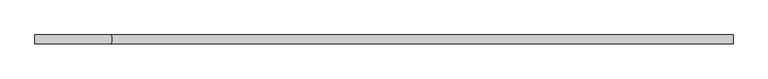
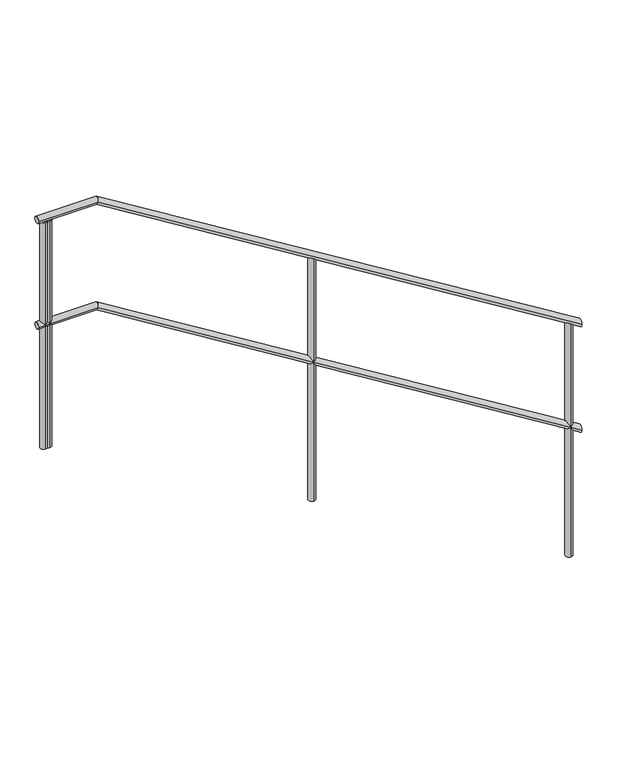
"""IFC4 building model written with IfcOpenShell, lengths in millimetres: railing geometry."""

import ifcopenshell
import ifcopenshell.guid

model = None  # the IFC model being written
_history = None  # IfcOwnerHistory: only IFC2X3 demands one
_inside = {}  # id of a spatial element -> (the spatial element, [elements in it])
_under = {}  # id of a project, library or spatial element -> (it, [spatial elements below it])
_declared = {}  # id of a project -> (the project, [libraries it declares])
_typed = {}  # id of a type object -> (the type object, [elements of that type])
_made_of = {}  # id of a material, layer set ... -> (it, [elements and type objects made of it])


def new_model(schema):
    """Start an empty IFC model of exactly this schema.

    Asked for "IFC4X3", IfcOpenShell would pick the latest addendum, in which some entities
    have other attributes; the version numbers below select the first issue.
    IFC2X3 requires an IfcOwnerHistory on every rooted entity: one is made here for all.
    """
    global model, _history
    if schema == "IFC4X3":
        model = ifcopenshell.file(schema_version=(4, 3, 0, 0))
    else:
        model = ifcopenshell.file(schema=schema)
    _inside.clear()
    _under.clear()
    _declared.clear()
    _typed.clear()
    _made_of.clear()
    _history = None
    if model.schema == "IFC2X3":
        org = make("IfcOrganization", Name="unknown")
        user = make(
            "IfcPersonAndOrganization",
            ThePerson=make("IfcPerson", FamilyName="unknown"),
            TheOrganization=org,
        )
        app = make(
            "IfcApplication",
            ApplicationDeveloper=org,
            Version="unknown",
            ApplicationFullName="unknown",
            ApplicationIdentifier="unknown",
        )
        _history = make(
            "IfcOwnerHistory",
            OwningUser=user,
            OwningApplication=app,
            ChangeAction="ADDED",
            CreationDate=0,
        )
    return model


def make(cls, **values):
    """One entity of the class cls with the attributes given. An attribute that is None is left unset."""
    return model.create_entity(
        cls, **{name: value for name, value in values.items() if value is not None}
    )


def rooted(cls, **values):
    """An entity with a GlobalId (a new one), such as an element, a storey or a relation."""
    return make(cls, GlobalId=ifcopenshell.guid.new(), OwnerHistory=_history, **values)


def si_unit(unit_type, name, prefix=None):
    """IfcSIUnit, for example si_unit("LENGTHUNIT", "METRE", prefix="MILLI")."""
    return make("IfcSIUnit", UnitType=unit_type, Prefix=prefix, Name=name)


def assignment(units):
    """IfcUnitAssignment: the units of a project."""
    return None if units is None else make("IfcUnitAssignment", Units=units)


def point(xyz):
    """IfcCartesianPoint."""
    return None if xyz is None else make("IfcCartesianPoint", Coordinates=xyz)


def direction(xyz):
    """IfcDirection."""
    return None if xyz is None else make("IfcDirection", DirectionRatios=xyz)


def frame(location, z_axis=None, x_axis=None):
    """IfcAxis2Placement3D, a coordinate frame: its origin and axes. An axis left out is left unset."""
    return make(
        "IfcAxis2Placement3D",
        Location=point(location),
        Axis=direction(z_axis),
        RefDirection=direction(x_axis),
    )


def frame_2d(location, x_axis=None):
    """IfcAxis2Placement2D, a coordinate frame in the plane: its origin and x axis."""
    return make(
        "IfcAxis2Placement2D", Location=point(location), RefDirection=direction(x_axis)
    )


def origin():
    """The frame at (0, 0, 0) with its axes left unset."""
    return frame((0.0, 0.0, 0.0))


def place(relative_to, where):
    """IfcLocalPlacement: puts the frame where relative to a parent placement (None: the world)."""
    return make(
        "IfcLocalPlacement", PlacementRelTo=relative_to, RelativePlacement=where
    )


def context(
    kind, dimensions, precision=None, world=None, true_north=None, identifier=None
):
    """IfcGeometricRepresentationContext, for example the 3D "Model" context."""
    return make(
        "IfcGeometricRepresentationContext",
        ContextIdentifier=identifier,
        ContextType=kind,
        CoordinateSpaceDimension=dimensions,
        Precision=precision,
        WorldCoordinateSystem=world,
        TrueNorth=true_north,
    )


def project(units=None, contexts=None):
    """IfcProject with its units and contexts."""
    return rooted(
        "IfcProject",
        Name="project",
        RepresentationContexts=contexts,
        UnitsInContext=assignment(units),
    )


def spatial(cls, under=None, at=None, **own):
    """A site, building, storey or space (cls), placed at a placement, below another one or the project."""
    s = rooted(cls, ObjectPlacement=at, **own)
    if under is not None:
        _under.setdefault(under.id(), (under, []))[1].append(s)
    return s


def circle_curve(where, radius):
    """IfcCircle in the frame where."""
    return make("IfcCircle", Position=where, Radius=radius)


def ellipse_curve(where, semi_axis1, semi_axis2):
    """IfcEllipse in the frame where."""
    return make(
        "IfcEllipse", Position=where, SemiAxis1=semi_axis1, SemiAxis2=semi_axis2
    )


def trimmed(basis, trim1, trim2, sense, master):
    """IfcTrimmedCurve: the piece of a basis curve between two trims."""
    return make(
        "IfcTrimmedCurve",
        BasisCurve=basis,
        Trim1=trim1,
        Trim2=trim2,
        SenseAgreement=sense,
        MasterRepresentation=master,
    )


def segment(curve, same_sense, transition):
    """IfcCompositeCurveSegment."""
    return make(
        "IfcCompositeCurveSegment",
        Transition=transition,
        SameSense=same_sense,
        ParentCurve=curve,
    )


def composite_curve(segments, self_intersect=None):
    """IfcCompositeCurve: segments joined end to end."""
    return make("IfcCompositeCurve", Segments=segments, SelfIntersect=self_intersect)


def outline(outer, holes=None, kind="AREA"):
    """IfcArbitraryClosedProfileDef: a profile drawn as a closed curve; with holes, ...WithVoids."""
    if holes is None:
        return make("IfcArbitraryClosedProfileDef", ProfileType=kind, OuterCurve=outer)
    return make(
        "IfcArbitraryProfileDefWithVoids",
        ProfileType=kind,
        OuterCurve=outer,
        InnerCurves=holes,
    )


def extrude(swept, where, along, depth):
    """IfcExtrudedAreaSolid: the profile swept, set in the frame where, extruded along a direction by depth."""
    return make(
        "IfcExtrudedAreaSolid",
        SweptArea=swept,
        Position=where,
        ExtrudedDirection=direction(along),
        Depth=depth,
    )


def shape(context_of_items, identifier, shape_type, items):
    """IfcShapeRepresentation: the items that make up one representation, for example the "Body"."""
    return make(
        "IfcShapeRepresentation",
        ContextOfItems=context_of_items,
        RepresentationIdentifier=identifier,
        RepresentationType=shape_type,
        Items=items,
    )


def source(mapping_origin, context_of_items, identifier, shape_type, items):
    """IfcRepresentationMap: a shape defined once, which mapped items show again and again."""
    return make(
        "IfcRepresentationMap",
        MappingOrigin=mapping_origin,
        MappedRepresentation=shape(context_of_items, identifier, shape_type, items),
    )


def transform(
    local_origin,
    x_axis=None,
    y_axis=None,
    z_axis=None,
    scale=None,
    scale2=None,
    scale3=None,
    uniform=True,
):
    """IfcCartesianTransformationOperator3D, or its non-uniform kind. x_axis, y_axis, z_axis: its Axis1, 2, 3."""
    if uniform:
        return make(
            "IfcCartesianTransformationOperator3D",
            Axis1=direction(x_axis),
            Axis2=direction(y_axis),
            LocalOrigin=point(local_origin),
            Scale=scale,
            Axis3=direction(z_axis),
        )
    return make(
        "IfcCartesianTransformationOperator3DnonUniform",
        Axis1=direction(x_axis),
        Axis2=direction(y_axis),
        LocalOrigin=point(local_origin),
        Scale=scale,
        Axis3=direction(z_axis),
        Scale2=scale2,
        Scale3=scale3,
    )


def mapped(mapping_source, mapping_target):
    """IfcMappedItem: shows the shape of a source again, moved by a transform."""
    return make(
        "IfcMappedItem", MappingSource=mapping_source, MappingTarget=mapping_target
    )


def made_of(thing, what):
    """Note that an element or type object is made of a material, layer set ...; save() writes the relation."""
    if what is not None:
        _made_of.setdefault(what.id(), (what, []))[1].append(thing)
    return thing


def element(
    cls,
    number,
    at=None,
    inside=None,
    cuts=None,
    type_object=None,
    material=None,
    context=None,
    identifier="Body",
    shape_type=None,
    held_by="IfcProductDefinitionShape",
    body=None,
    shapes=None,
    **own,
):
    """One element of the class cls, such as IfcWall. Its Tag is "e" and its number.

    at: its placement. inside: the storey or other place that contains it. cuts: it is an
    opening in that element (IfcRelVoidsElement). A single representation is given by context,
    identifier, shape_type and body (its items); several are given by shapes. held_by: the class
    of the entity that holds the representations. save() writes the other relations.
    """
    e = rooted(cls, Tag="e%d" % number, ObjectPlacement=at, **own)
    if body is not None:
        shapes = [shape(context, identifier, shape_type, body)]
    if shapes is not None:
        e.Representation = make(held_by, Representations=shapes)
    if inside is not None:
        _inside.setdefault(inside.id(), (inside, []))[1].append(e)
    if cuts is not None:
        rooted(
            "IfcRelVoidsElement", RelatingBuildingElement=cuts, RelatedOpeningElement=e
        )
    if type_object is not None:
        _typed.setdefault(type_object.id(), (type_object, []))[1].append(e)
    return made_of(e, material)


def aggregate(whole, parts):
    """IfcRelAggregates: a whole, such as a stair, and the parts it consists of."""
    return rooted("IfcRelAggregates", RelatingObject=whole, RelatedObjects=parts)


def save(model, path):
    """Write the relations noted so far, then the file.

    IfcRelAggregates (storeys below a building ...), IfcRelContainedInSpatialStructure (elements
    in a storey), IfcRelDefinesByType, IfcRelAssociatesMaterial and IfcRelDeclares: one each for
    every whole, place, type object, material and project.
    """
    for whole, parts in _under.values():
        aggregate(whole, parts)
    for where, things in _inside.values():
        rooted(
            "IfcRelContainedInSpatialStructure",
            RelatedElements=things,
            RelatingStructure=where,
        )
    for kind, things in _typed.values():
        rooted("IfcRelDefinesByType", RelatedObjects=things, RelatingType=kind)
    for what, things in _made_of.values():
        rooted("IfcRelAssociatesMaterial", RelatedObjects=things, RelatingMaterial=what)
    for by, libraries in _declared.values():
        rooted("IfcRelDeclares", RelatingContext=by, RelatedDefinitions=libraries)
    model.write(path)


def plane_surface(at):
    """IfcPlane: the flat surface through the origin of the frame at, square to its z axis."""
    return make("IfcPlane", Position=at)


def cylinder_surface(at, radius):
    """IfcCylindricalSurface: all points at the distance radius from the z axis of the frame at."""
    return make("IfcCylindricalSurface", Position=at, Radius=radius)


def advanced_brep(points, edges, surfaces, faces):
    """IfcAdvancedBrep: a solid bounded by faces that lie on surfaces and meet in shared edges.

    An edge is (start, end): straight between two places in points (the first is 0);
    or (start, end, curve); or (start, end, curve, False) where it runs against its curve.
    A face is (place in surfaces, loops), or (place, loops, False) where it looks against
    its surface's normal. A loop lists edges by number (the first is 1), with a minus sign
    where the edge is run from its end to its start. The first loop is the outer one.
    """
    corners = [point(p) for p in points]
    vertices = [make("IfcVertexPoint", VertexGeometry=c) for c in corners]
    made = []
    for start, end, *more in edges:
        made.append(
            make(
                "IfcEdgeCurve",
                EdgeStart=vertices[start],
                EdgeEnd=vertices[end],
                EdgeGeometry=more[0] if more else make("IfcPolyline", Points=[corners[start], corners[end]]),
                SameSense=more[1] if len(more) > 1 else True,
            )
        )
    hull = []
    for where, loops, *sense in faces:
        bounds = []
        for j, loop in enumerate(loops):
            ring = [make("IfcOrientedEdge", EdgeElement=made[abs(k) - 1], Orientation=k > 0) for k in loop]
            bounds.append(
                make(
                    "IfcFaceOuterBound" if j == 0 else "IfcFaceBound",
                    Bound=make("IfcEdgeLoop", EdgeList=ring),
                    Orientation=True,
                )
            )
        hull.append(make("IfcAdvancedFace", Bounds=bounds, FaceSurface=surfaces[where], SameSense=sense[0] if sense else True))
    return make("IfcAdvancedBrep", Outer=make("IfcClosedShell", CfsFaces=hull))


def railing_16da177b(model_context):
    return source(origin(), model_context, "Body", "SolidModel", [
        advanced_brep(
        [(6405.7243044, 63987.0208589, -450.9609787), (6405.7243044, 64017.0208589, -450.9609787), (4241.4675189, 63987.0208589, 885.0), (4241.4675189, 64017.0208589, 885.0), (3975.7243044, 63987.0208589, 885.0), (3975.7243044, 64017.0208589, 885.0)],
        [
            (0, 1, ellipse_curve(frame((6405.7243044, 64002.0208589, -450.9609787), z_axis=(1.0, 0.0, 0.0), x_axis=(0.0, 0.0, -1.0)), 17.6276454, 15.0)),
            (1, 0, ellipse_curve(frame((6405.7243044, 64002.0208589, -450.9609787), z_axis=(1.0, 0.0, 0.0), x_axis=(0.0, 0.0, -1.0)), 17.6276454, 15.0)),
            (0, 2),
            (2, 3, ellipse_curve(frame((4241.4675189, 64002.0208589, 885.0), z_axis=(0.9620125025549408, 0.0, -0.2730053935877092), x_axis=(-0.2730053935877087, 0.0, -0.962012502554941)), 15.5923129, 15.0)),
            (3, 1),
            (3, 2, ellipse_curve(frame((4241.4675189, 64002.0208589, 885.0), z_axis=(0.9620125025549408, 0.0, -0.2730053935877092), x_axis=(-0.2730053935877087, 0.0, -0.962012502554941)), 15.5923129, 15.0)),
            (4, 5, circle_curve(frame((3975.7243044, 64002.0208589, 885.0), z_axis=(-1.0, 0.0, 0.0), x_axis=(0.0, 1.0, 0.0)), 15.0)),
            (5, 4, circle_curve(frame((3975.7243044, 64002.0208589, 885.0), z_axis=(-1.0, 0.0, 0.0), x_axis=(0.0, 1.0, 0.0)), 15.0)),
            (2, 4),
            (5, 3),
        ],
        [
            plane_surface(frame((6405.7243044, 64002.0208589, -433.3333333), z_axis=(1.0, 0.0, 0.0), x_axis=(0.0, -1.0, 0.0))),
            cylinder_surface(frame((6397.8452664, 64002.0208589, -446.097375), z_axis=(0.8509361101440399, 0.0, -0.5252692037926174), x_axis=(0.0, 1.0, 0.0)), 15.0),
            plane_surface(frame((3975.7243044, 64002.0208589, 900.0), z_axis=(-1.0, 0.0, 0.0), x_axis=(0.0, -1.0, 0.0))),
            cylinder_surface(frame((4245.7243044, 64002.0208589, 885.0), z_axis=(1.0, 0.0, 0.0), x_axis=(0.0, 1.0, 0.0)), 15.0),
        ],
        [
            (0, [[1, 2]]),
            (1, [[-1, 3, 4, 5]]),
            (1, [[-2, -5, 6, -3]]),
            (2, [[7, 8]]),
            (3, [[-4, 9, -8, 10]]),
            (3, [[-6, -10, -7, -9]]),
        ],
    ),
        advanced_brep(
        [(6405.7243044, 63987.0208589, 49.0390213), (6405.7243044, 64017.0208589, 49.0390213), (4241.4675189, 63987.0208589, 1385.0), (4241.4675189, 64017.0208589, 1385.0), (3975.7243044, 63987.0208589, 1385.0), (3975.7243044, 64017.0208589, 1385.0)],
        [
            (0, 1, ellipse_curve(frame((6405.7243044, 64002.0208589, 49.0390213), z_axis=(1.0, 0.0, 0.0), x_axis=(0.0, 0.0, -1.0)), 17.6276454, 15.0)),
            (1, 0, ellipse_curve(frame((6405.7243044, 64002.0208589, 49.0390213), z_axis=(1.0, 0.0, 0.0), x_axis=(0.0, 0.0, -1.0)), 17.6276454, 15.0)),
            (0, 2),
            (2, 3, ellipse_curve(frame((4241.4675189, 64002.0208589, 1385.0), z_axis=(0.9620125025549408, 0.0, -0.2730053935877092), x_axis=(-0.2730053935877087, 0.0, -0.962012502554941)), 15.5923129, 15.0)),
            (3, 1),
            (3, 2, ellipse_curve(frame((4241.4675189, 64002.0208589, 1385.0), z_axis=(0.9620125025549408, 0.0, -0.2730053935877092), x_axis=(-0.2730053935877087, 0.0, -0.962012502554941)), 15.5923129, 15.0)),
            (4, 5, circle_curve(frame((3975.7243044, 64002.0208589, 1385.0), z_axis=(-1.0, 0.0, 0.0), x_axis=(0.0, 1.0, 0.0)), 15.0)),
            (5, 4, circle_curve(frame((3975.7243044, 64002.0208589, 1385.0), z_axis=(-1.0, 0.0, 0.0), x_axis=(0.0, 1.0, 0.0)), 15.0)),
            (2, 4),
            (5, 3),
        ],
        [
            plane_surface(frame((6405.7243044, 64002.0208589, 66.6666667), z_axis=(1.0, 0.0, 0.0), x_axis=(0.0, -1.0, 0.0))),
            cylinder_surface(frame((6397.8452664, 64002.0208589, 53.902625), z_axis=(0.8509361101440399, 0.0, -0.5252692037926174), x_axis=(0.0, 1.0, 0.0)), 15.0),
            plane_surface(frame((3975.7243044, 64002.0208589, 1400.0), z_axis=(-1.0, 0.0, 0.0), x_axis=(0.0, -1.0, 0.0))),
            cylinder_surface(frame((4245.7243044, 64002.0208589, 1385.0), z_axis=(1.0, 0.0, 0.0), x_axis=(0.0, 1.0, 0.0)), 15.0),
        ],
        [
            (0, [[1, 2]]),
            (1, [[-1, 3, 4, 5]]),
            (1, [[-2, -5, 6, -3]]),
            (2, [[7, 8]]),
            (3, [[-4, 9, -8, 10]]),
            (3, [[-6, -10, -7, -9]]),
        ],
    ),
        extrude(outline(composite_curve([segment(trimmed(circle_curve(frame_2d((4005.7243044, 64002.0208589)), 15.0), [point((4005.7243044, 63987.0208589))], [point((4005.7243044, 64017.0208589))], False, "CARTESIAN"), True, "CONTINUOUS"), segment(trimmed(circle_curve(frame_2d((4005.7243044, 64002.0208589)), 15.0), [point((4005.7243044, 64017.0208589))], [point((4005.7243044, 63987.0208589))], False, "CARTESIAN"), True, "CONTINUOUS")], self_intersect=False)), frame((0.0, 0.0, 300.0), z_axis=(0.0, 0.0, 1.0), x_axis=(1.0, 0.0, 0.0)), (0.0, 0.0, 1.0), 1070.0),
        advanced_brep(
        [(5205.7243044, 64017.0208589, 777.4074074), (5205.7243044, 64017.0208589, -366.6666667), (5205.7243044, 63987.0208589, -366.6666667), (5205.7243044, 63987.0208589, 777.4074074)],
        [
            (0, 1),
            (1, 2, circle_curve(frame((5205.7243044, 64002.0208589, -366.6666667), z_axis=(0.0, 0.0, 1.0), x_axis=(0.0, -1.0, 0.0)), 15.0)),
            (2, 3),
            (3, 0, ellipse_curve(frame((5205.7243044, 64002.0208589, 777.4074074), z_axis=(-0.5252692037926167, 0.0, -0.8509361101440406), x_axis=(-0.8509361101440406, 0.0, 0.5252692037926162)), 17.6276454, 15.0)),
            (0, 3, ellipse_curve(frame((5205.7243044, 64002.0208589, 777.4074074), z_axis=(-0.5252692037926167, 0.0, -0.8509361101440406), x_axis=(-0.8509361101440406, 0.0, 0.5252692037926162)), 17.6276454, 15.0)),
            (2, 1, circle_curve(frame((5205.7243044, 64002.0208589, -366.6666667), z_axis=(0.0, 0.0, 1.0), x_axis=(0.0, -1.0, 0.0)), 15.0)),
        ],
        [
            cylinder_surface(frame((5205.7243044, 64002.0208589, -466.6666667), z_axis=(0.0, 0.0, 1.0), x_axis=(0.0, -1.0, 0.0)), 15.0),
            plane_surface(frame((5180.7243044, 63977.0208589, 792.8395062), z_axis=(0.5252692037926167, 0.0, 0.8509361101440406), x_axis=(0.0, 1.0, 0.0))),
            plane_surface(frame((5230.7243044, 63977.0208589, -366.6666667), z_axis=(0.0, 0.0, -1.0), x_axis=(0.0, 1.0, 0.0))),
        ],
        [
            (0, [[1, 2, 3, 4]]),
            (0, [[-1, 5, -3, 6]]),
            (1, [[-4, -5]]),
            (2, [[-2, -6]]),
        ],
    ),
        extrude(outline(composite_curve([segment(trimmed(circle_curve(frame_2d((4025.7243044, 64002.0208589)), 15.0), [point((4025.7243044, 63987.0208589))], [point((4025.7243044, 64017.0208589))], False, "CARTESIAN"), True, "CONTINUOUS"), segment(trimmed(circle_curve(frame_2d((4025.7243044, 64002.0208589)), 15.0), [point((4025.7243044, 64017.0208589))], [point((4025.7243044, 63987.0208589))], False, "CARTESIAN"), True, "CONTINUOUS")], self_intersect=False)), frame((0.0, 0.0, 300.0), z_axis=(0.0, 0.0, 1.0), x_axis=(1.0, 0.0, 0.0)), (0.0, 0.0, 1.0), 1070.0),
        advanced_brep(
        [(6355.7243044, 64017.0208589, 67.5308642), (6355.7243044, 64017.0208589, -1033.3333333), (6355.7243044, 63987.0208589, -1033.3333333), (6355.7243044, 63987.0208589, 67.5308642)],
        [
            (0, 1),
            (1, 2, circle_curve(frame((6355.7243044, 64002.0208589, -1033.3333333), z_axis=(0.0, 0.0, 1.0), x_axis=(0.0, -1.0, 0.0)), 15.0)),
            (2, 3),
            (3, 0, ellipse_curve(frame((6355.7243044, 64002.0208589, 67.5308642), z_axis=(-0.5252692037926167, 0.0, -0.8509361101440406), x_axis=(-0.8509361101440406, 0.0, 0.5252692037926162)), 17.6276454, 15.0)),
            (0, 3, ellipse_curve(frame((6355.7243044, 64002.0208589, 67.5308642), z_axis=(-0.5252692037926167, 0.0, -0.8509361101440406), x_axis=(-0.8509361101440406, 0.0, 0.5252692037926162)), 17.6276454, 15.0)),
            (2, 1, circle_curve(frame((6355.7243044, 64002.0208589, -1033.3333333), z_axis=(0.0, 0.0, 1.0), x_axis=(0.0, -1.0, 0.0)), 15.0)),
        ],
        [
            cylinder_surface(frame((6355.7243044, 64002.0208589, -1133.3333333), z_axis=(0.0, 0.0, 1.0), x_axis=(0.0, -1.0, 0.0)), 15.0),
            plane_surface(frame((6330.7243044, 63977.0208589, 82.962963), z_axis=(0.5252692037926167, 0.0, 0.8509361101440406), x_axis=(0.0, 1.0, 0.0))),
            plane_surface(frame((6380.7243044, 63977.0208589, -1033.3333333), z_axis=(0.0, 0.0, -1.0), x_axis=(0.0, 1.0, 0.0))),
        ],
        [
            (0, [[1, 2, 3, 4]]),
            (0, [[-1, 5, -3, 6]]),
            (1, [[-4, -5]]),
            (2, [[-2, -6]]),
        ],
    ),
    ])


if __name__ == "__main__":
    model = new_model("IFC4")
    model_context = context("Model", 3, world=origin())
    ifc_project = project(units=[si_unit("LENGTHUNIT", "METRE", prefix="MILLI")], contexts=[model_context])
    site = spatial("IfcSite", under=ifc_project)
    building = spatial("IfcBuilding", under=site)
    placement = place(None, origin())
    railing_shape = railing_16da177b(model_context)
    element("IfcRailing", 1, at=placement, inside=building, context=model_context, shape_type="MappedRepresentation", body=[
        mapped(railing_shape, transform((0.0, 0.0, 0.0), x_axis=(1.0, 0.0, 0.0), y_axis=(0.0, 1.0, 0.0), z_axis=(0.0, 0.0, 1.0))),
    ])
    save(model, "model.ifc")
